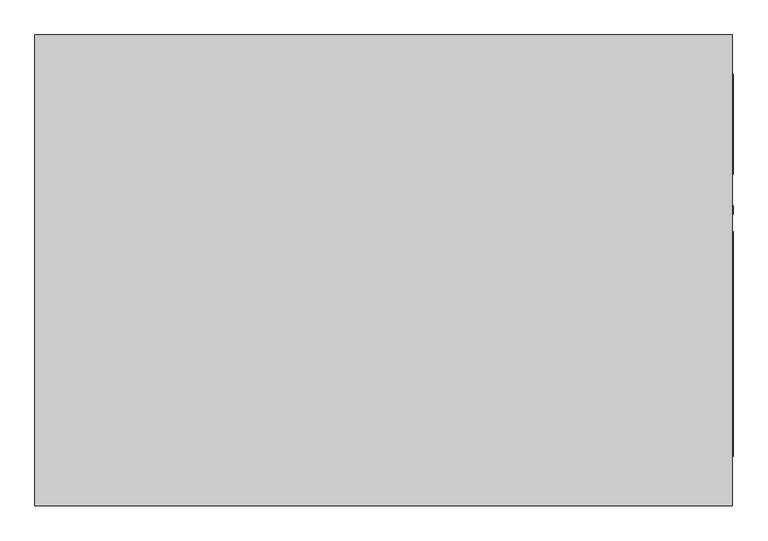
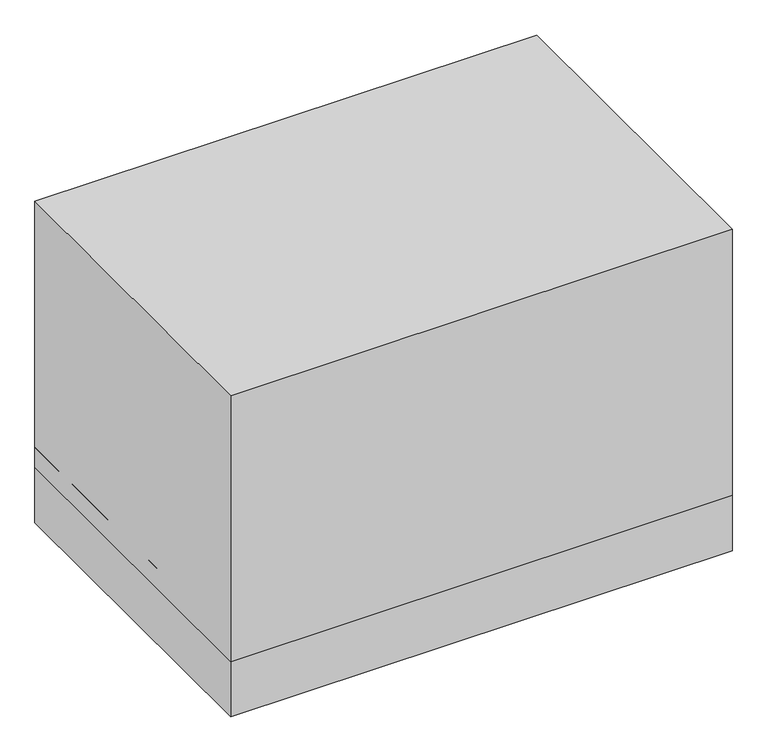
"""IFC4 building model written with IfcOpenShell, lengths in millimetres: proxy geometry, Carrier_48TC_Standard_Efficiency_Gas_Heat_Electric_Cooling_Packaged_Rooftop_Unit_3_to_15_nominal_tons : 12.5 ton 48TC**14."""

import ifcopenshell
import ifcopenshell.guid

model = None  # the IFC model being written
_history = None  # IfcOwnerHistory: only IFC2X3 demands one
_inside = {}  # id of a spatial element -> (the spatial element, [elements in it])
_under = {}  # id of a project, library or spatial element -> (it, [spatial elements below it])
_declared = {}  # id of a project -> (the project, [libraries it declares])
_typed = {}  # id of a type object -> (the type object, [elements of that type])
_made_of = {}  # id of a material, layer set ... -> (it, [elements and type objects made of it])


def new_model(schema):
    """Start an empty IFC model of exactly this schema.

    Asked for "IFC4X3", IfcOpenShell would pick the latest addendum, in which some entities
    have other attributes; the version numbers below select the first issue.
    IFC2X3 requires an IfcOwnerHistory on every rooted entity: one is made here for all.
    """
    global model, _history
    if schema == "IFC4X3":
        model = ifcopenshell.file(schema_version=(4, 3, 0, 0))
    else:
        model = ifcopenshell.file(schema=schema)
    _inside.clear()
    _under.clear()
    _declared.clear()
    _typed.clear()
    _made_of.clear()
    _history = None
    if model.schema == "IFC2X3":
        org = make("IfcOrganization", Name="unknown")
        user = make(
            "IfcPersonAndOrganization",
            ThePerson=make("IfcPerson", FamilyName="unknown"),
            TheOrganization=org,
        )
        app = make(
            "IfcApplication",
            ApplicationDeveloper=org,
            Version="unknown",
            ApplicationFullName="unknown",
            ApplicationIdentifier="unknown",
        )
        _history = make(
            "IfcOwnerHistory",
            OwningUser=user,
            OwningApplication=app,
            ChangeAction="ADDED",
            CreationDate=0,
        )
    return model


def make(cls, **values):
    """One entity of the class cls with the attributes given. An attribute that is None is left unset."""
    return model.create_entity(
        cls, **{name: value for name, value in values.items() if value is not None}
    )


def rooted(cls, **values):
    """An entity with a GlobalId (a new one), such as an element, a storey or a relation."""
    return make(cls, GlobalId=ifcopenshell.guid.new(), OwnerHistory=_history, **values)


def si_unit(unit_type, name, prefix=None):
    """IfcSIUnit, for example si_unit("LENGTHUNIT", "METRE", prefix="MILLI")."""
    return make("IfcSIUnit", UnitType=unit_type, Prefix=prefix, Name=name)


def assignment(units):
    """IfcUnitAssignment: the units of a project."""
    return None if units is None else make("IfcUnitAssignment", Units=units)


def point(xyz):
    """IfcCartesianPoint."""
    return None if xyz is None else make("IfcCartesianPoint", Coordinates=xyz)


def direction(xyz):
    """IfcDirection."""
    return None if xyz is None else make("IfcDirection", DirectionRatios=xyz)


def frame(location, z_axis=None, x_axis=None):
    """IfcAxis2Placement3D, a coordinate frame: its origin and axes. An axis left out is left unset."""
    return make(
        "IfcAxis2Placement3D",
        Location=point(location),
        Axis=direction(z_axis),
        RefDirection=direction(x_axis),
    )


def frame_2d(location, x_axis=None):
    """IfcAxis2Placement2D, a coordinate frame in the plane: its origin and x axis."""
    return make(
        "IfcAxis2Placement2D", Location=point(location), RefDirection=direction(x_axis)
    )


def origin():
    """The frame at (0, 0, 0) with its axes left unset."""
    return frame((0.0, 0.0, 0.0))


def origin_with_axes():
    """The frame at (0, 0, 0) with the z axis (0, 0, 1) and the x axis (1, 0, 0) written out."""
    return frame((0.0, 0.0, 0.0), z_axis=(0.0, 0.0, 1.0), x_axis=(1.0, 0.0, 0.0))


def place(relative_to, where):
    """IfcLocalPlacement: puts the frame where relative to a parent placement (None: the world)."""
    return make(
        "IfcLocalPlacement", PlacementRelTo=relative_to, RelativePlacement=where
    )


def context(
    kind, dimensions, precision=None, world=None, true_north=None, identifier=None
):
    """IfcGeometricRepresentationContext, for example the 3D "Model" context."""
    return make(
        "IfcGeometricRepresentationContext",
        ContextIdentifier=identifier,
        ContextType=kind,
        CoordinateSpaceDimension=dimensions,
        Precision=precision,
        WorldCoordinateSystem=world,
        TrueNorth=true_north,
    )


def project(units=None, contexts=None):
    """IfcProject with its units and contexts."""
    return rooted(
        "IfcProject",
        Name="project",
        RepresentationContexts=contexts,
        UnitsInContext=assignment(units),
    )


def spatial(cls, under=None, at=None, **own):
    """A site, building, storey or space (cls), placed at a placement, below another one or the project."""
    s = rooted(cls, ObjectPlacement=at, **own)
    if under is not None:
        _under.setdefault(under.id(), (under, []))[1].append(s)
    return s


def polyline(points):
    """IfcPolyline through the points."""
    return make("IfcPolyline", Points=[point(p) for p in points])


def circle_curve(where, radius):
    """IfcCircle in the frame where."""
    return make("IfcCircle", Position=where, Radius=radius)


def trimmed(basis, trim1, trim2, sense, master):
    """IfcTrimmedCurve: the piece of a basis curve between two trims."""
    return make(
        "IfcTrimmedCurve",
        BasisCurve=basis,
        Trim1=trim1,
        Trim2=trim2,
        SenseAgreement=sense,
        MasterRepresentation=master,
    )


def segment(curve, same_sense, transition):
    """IfcCompositeCurveSegment."""
    return make(
        "IfcCompositeCurveSegment",
        Transition=transition,
        SameSense=same_sense,
        ParentCurve=curve,
    )


def composite_curve(segments, self_intersect=None):
    """IfcCompositeCurve: segments joined end to end."""
    return make("IfcCompositeCurve", Segments=segments, SelfIntersect=self_intersect)


def outline(outer, holes=None, kind="AREA"):
    """IfcArbitraryClosedProfileDef: a profile drawn as a closed curve; with holes, ...WithVoids."""
    if holes is None:
        return make("IfcArbitraryClosedProfileDef", ProfileType=kind, OuterCurve=outer)
    return make(
        "IfcArbitraryProfileDefWithVoids",
        ProfileType=kind,
        OuterCurve=outer,
        InnerCurves=holes,
    )


def extrude(swept, where, along, depth):
    """IfcExtrudedAreaSolid: the profile swept, set in the frame where, extruded along a direction by depth."""
    return make(
        "IfcExtrudedAreaSolid",
        SweptArea=swept,
        Position=where,
        ExtrudedDirection=direction(along),
        Depth=depth,
    )


def shape(context_of_items, identifier, shape_type, items):
    """IfcShapeRepresentation: the items that make up one representation, for example the "Body"."""
    return make(
        "IfcShapeRepresentation",
        ContextOfItems=context_of_items,
        RepresentationIdentifier=identifier,
        RepresentationType=shape_type,
        Items=items,
    )


def source(mapping_origin, context_of_items, identifier, shape_type, items):
    """IfcRepresentationMap: a shape defined once, which mapped items show again and again."""
    return make(
        "IfcRepresentationMap",
        MappingOrigin=mapping_origin,
        MappedRepresentation=shape(context_of_items, identifier, shape_type, items),
    )


def transform(
    local_origin,
    x_axis=None,
    y_axis=None,
    z_axis=None,
    scale=None,
    scale2=None,
    scale3=None,
    uniform=True,
):
    """IfcCartesianTransformationOperator3D, or its non-uniform kind. x_axis, y_axis, z_axis: its Axis1, 2, 3."""
    if uniform:
        return make(
            "IfcCartesianTransformationOperator3D",
            Axis1=direction(x_axis),
            Axis2=direction(y_axis),
            LocalOrigin=point(local_origin),
            Scale=scale,
            Axis3=direction(z_axis),
        )
    return make(
        "IfcCartesianTransformationOperator3DnonUniform",
        Axis1=direction(x_axis),
        Axis2=direction(y_axis),
        LocalOrigin=point(local_origin),
        Scale=scale,
        Axis3=direction(z_axis),
        Scale2=scale2,
        Scale3=scale3,
    )


def mapped(mapping_source, mapping_target):
    """IfcMappedItem: shows the shape of a source again, moved by a transform."""
    return make(
        "IfcMappedItem", MappingSource=mapping_source, MappingTarget=mapping_target
    )


def made_of(thing, what):
    """Note that an element or type object is made of a material, layer set ...; save() writes the relation."""
    if what is not None:
        _made_of.setdefault(what.id(), (what, []))[1].append(thing)
    return thing


def element(
    cls,
    number,
    at=None,
    inside=None,
    cuts=None,
    type_object=None,
    material=None,
    context=None,
    identifier="Body",
    shape_type=None,
    held_by="IfcProductDefinitionShape",
    body=None,
    shapes=None,
    **own,
):
    """One element of the class cls, such as IfcWall. Its Tag is "e" and its number.

    at: its placement. inside: the storey or other place that contains it. cuts: it is an
    opening in that element (IfcRelVoidsElement). A single representation is given by context,
    identifier, shape_type and body (its items); several are given by shapes. held_by: the class
    of the entity that holds the representations. save() writes the other relations.
    """
    e = rooted(cls, Tag="e%d" % number, ObjectPlacement=at, **own)
    if body is not None:
        shapes = [shape(context, identifier, shape_type, body)]
    if shapes is not None:
        e.Representation = make(held_by, Representations=shapes)
    if inside is not None:
        _inside.setdefault(inside.id(), (inside, []))[1].append(e)
    if cuts is not None:
        rooted(
            "IfcRelVoidsElement", RelatingBuildingElement=cuts, RelatedOpeningElement=e
        )
    if type_object is not None:
        _typed.setdefault(type_object.id(), (type_object, []))[1].append(e)
    return made_of(e, material)


def aggregate(whole, parts):
    """IfcRelAggregates: a whole, such as a stair, and the parts it consists of."""
    return rooted("IfcRelAggregates", RelatingObject=whole, RelatedObjects=parts)


def save(model, path):
    """Write the relations noted so far, then the file.

    IfcRelAggregates (storeys below a building ...), IfcRelContainedInSpatialStructure (elements
    in a storey), IfcRelDefinesByType, IfcRelAssociatesMaterial and IfcRelDeclares: one each for
    every whole, place, type object, material and project.
    """
    for whole, parts in _under.values():
        aggregate(whole, parts)
    for where, things in _inside.values():
        rooted(
            "IfcRelContainedInSpatialStructure",
            RelatedElements=things,
            RelatingStructure=where,
        )
    for kind, things in _typed.values():
        rooted("IfcRelDefinesByType", RelatedObjects=things, RelatingType=kind)
    for what, things in _made_of.values():
        rooted("IfcRelAssociatesMaterial", RelatedObjects=things, RelatingMaterial=what)
    for by, libraries in _declared.values():
        rooted("IfcRelDeclares", RelatingContext=by, RelatedDefinitions=libraries)
    model.write(path)


def plane_surface(at):
    """IfcPlane: the flat surface through the origin of the frame at, square to its z axis."""
    return make("IfcPlane", Position=at)


def revolved_surface(curve, axis_point, axis_direction):
    """IfcSurfaceOfRevolution: the curve turned about the line through axis_point along axis_direction."""
    return make(
        "IfcSurfaceOfRevolution",
        SweptCurve=make("IfcArbitraryOpenProfileDef", ProfileType="CURVE", Curve=curve),
        AxisPosition=make("IfcAxis1Placement", Location=point(axis_point), Axis=direction(axis_direction)),
    )


def advanced_brep(points, edges, surfaces, faces):
    """IfcAdvancedBrep: a solid bounded by faces that lie on surfaces and meet in shared edges.

    An edge is (start, end): straight between two places in points (the first is 0);
    or (start, end, curve); or (start, end, curve, False) where it runs against its curve.
    A face is (place in surfaces, loops), or (place, loops, False) where it looks against
    its surface's normal. A loop lists edges by number (the first is 1), with a minus sign
    where the edge is run from its end to its start. The first loop is the outer one.
    """
    corners = [point(p) for p in points]
    vertices = [make("IfcVertexPoint", VertexGeometry=c) for c in corners]
    made = []
    for start, end, *more in edges:
        made.append(
            make(
                "IfcEdgeCurve",
                EdgeStart=vertices[start],
                EdgeEnd=vertices[end],
                EdgeGeometry=more[0] if more else make("IfcPolyline", Points=[corners[start], corners[end]]),
                SameSense=more[1] if len(more) > 1 else True,
            )
        )
    hull = []
    for where, loops, *sense in faces:
        bounds = []
        for j, loop in enumerate(loops):
            ring = [make("IfcOrientedEdge", EdgeElement=made[abs(k) - 1], Orientation=k > 0) for k in loop]
            bounds.append(
                make(
                    "IfcFaceOuterBound" if j == 0 else "IfcFaceBound",
                    Bound=make("IfcEdgeLoop", EdgeList=ring),
                    Orientation=True,
                )
            )
        hull.append(make("IfcAdvancedFace", Bounds=bounds, FaceSurface=surfaces[where], SameSense=sense[0] if sense else True))
    return make("IfcAdvancedBrep", Outer=make("IfcClosedShell", CfsFaces=hull))


def mechanical_equipment_3d4f0b1e(model_context):
    return source(origin(), model_context, "Body", "SolidModel", [
        extrude(outline(composite_curve([segment(trimmed(circle_curve(frame_2d((193.675, 438.15)), 13.2953125), [point((180.3796875, 438.15))], [point((206.9703125, 438.15))], False, "CARTESIAN"), True, "CONTINUOUS"), segment(trimmed(circle_curve(frame_2d((193.675, 438.15)), 13.2953125), [point((206.9703125, 438.15))], [point((180.3796875, 438.15))], False, "CARTESIAN"), True, "CONTINUOUS")], self_intersect=False)), frame((1119.1875, 0.0, 0.0), z_axis=(1.0, 0.0, 0.0), x_axis=(0.0, 1.0, 0.0)), (0.0, 0.0, 1.0), 3.175),
        advanced_brep(
        [(1119.1875, 755.65, 1514.475), (-1119.1875, 755.65, 1514.475), (-1119.1875, -755.65, 1514.475), (1119.1875, -755.65, 1514.475), (1119.1875, 755.65, 260.35), (1119.1875, -755.65, 260.35), (-1119.1875, -755.65, 260.35), (-1119.1875, 755.65, 260.35), (1036.6375, -596.9, 260.35), (1036.6375, 0.0, 260.35), (681.0375, 0.0, 260.35), (681.0375, -596.9, 260.35), (1036.6375, 590.55, 260.35), (112.7125, 590.55, 260.35), (112.7125, 269.875, 260.35), (1036.6375, 269.875, 260.35), (176.8078125, -107.95, 260.35), (150.2171875, -107.95, 260.35), (-355.6, -476.25, 260.35), (-377.825, -476.25, 260.35), (-344.4875, -349.25, 260.35), (-388.9375, -349.25, 260.35), (-344.4875, -298.45, 260.35), (-388.9375, -298.45, 260.35), (1036.6375, -596.9, 381.0), (681.0375, -596.9, 381.0), (681.0375, 0.0, 381.0), (1036.6375, 0.0, 381.0), (1036.6375, 590.55, 381.0), (1036.6375, 269.875, 381.0), (112.7125, 269.875, 381.0), (112.7125, 590.55, 381.0), (176.8078125, -107.95, 406.4), (150.2171875, -107.95, 406.4), (-355.6, -476.25, 406.4), (-377.825, -476.25, 406.4), (-344.4875, -349.25, 406.4), (-388.9375, -349.25, 406.4), (-344.4875, -298.45, 406.4), (-388.9375, -298.45, 406.4)],
        [
            (0, 1),
            (1, 2),
            (2, 3),
            (3, 0),
            (4, 5),
            (5, 6),
            (6, 7),
            (7, 4),
            (8, 9),
            (9, 10),
            (10, 11),
            (11, 8),
            (12, 13),
            (13, 14),
            (14, 15),
            (15, 12),
            (16, 17, circle_curve(frame((163.5125, -107.95, 260.35), z_axis=(0.0, 0.0, 1.0), x_axis=(-1.0, 0.0, 0.0)), 13.2953125)),
            (17, 16, circle_curve(frame((163.5125, -107.95, 260.35), z_axis=(0.0, 0.0, 1.0), x_axis=(-1.0, 0.0, 0.0)), 13.2953125)),
            (18, 19, circle_curve(frame((-366.7125, -476.25, 260.35), z_axis=(0.0, 0.0, 1.0), x_axis=(-1.0, 0.0, 0.0)), 11.1125)),
            (19, 18, circle_curve(frame((-366.7125, -476.25, 260.35), z_axis=(0.0, 0.0, 1.0), x_axis=(-1.0, 0.0, 0.0)), 11.1125)),
            (20, 21, circle_curve(frame((-366.7125, -349.25, 260.35), z_axis=(0.0, 0.0, 1.0), x_axis=(-1.0, 0.0, 0.0)), 22.225)),
            (21, 20, circle_curve(frame((-366.7125, -349.25, 260.35), z_axis=(0.0, 0.0, 1.0), x_axis=(-1.0, 0.0, 0.0)), 22.225)),
            (22, 23, circle_curve(frame((-366.7125, -298.45, 260.35), z_axis=(0.0, 0.0, 1.0), x_axis=(-1.0, 0.0, 0.0)), 22.225)),
            (23, 22, circle_curve(frame((-366.7125, -298.45, 260.35), z_axis=(0.0, 0.0, 1.0), x_axis=(-1.0, 0.0, 0.0)), 22.225)),
            (0, 4),
            (7, 1),
            (6, 2),
            (5, 3),
            (24, 25),
            (25, 26),
            (26, 27),
            (27, 24),
            (27, 9),
            (8, 24),
            (26, 10),
            (25, 11),
            (28, 29),
            (29, 30),
            (30, 31),
            (31, 28),
            (31, 13),
            (12, 28),
            (30, 14),
            (29, 15),
            (32, 33, circle_curve(frame((163.5125, -107.95, 406.4), z_axis=(0.0, 0.0, -1.0), x_axis=(-1.0, 0.0, 0.0)), 13.2953125)),
            (33, 32, circle_curve(frame((163.5125, -107.95, 406.4), z_axis=(0.0, 0.0, -1.0), x_axis=(-1.0, 0.0, 0.0)), 13.2953125)),
            (33, 17),
            (16, 32),
            (34, 35, circle_curve(frame((-366.7125, -476.25, 406.4), z_axis=(0.0, 0.0, -1.0), x_axis=(-1.0, 0.0, 0.0)), 11.1125)),
            (35, 34, circle_curve(frame((-366.7125, -476.25, 406.4), z_axis=(0.0, 0.0, -1.0), x_axis=(-1.0, 0.0, 0.0)), 11.1125)),
            (35, 19),
            (18, 34),
            (36, 37, circle_curve(frame((-366.7125, -349.25, 406.4), z_axis=(0.0, 0.0, -1.0), x_axis=(-1.0, 0.0, 0.0)), 22.225)),
            (37, 36, circle_curve(frame((-366.7125, -349.25, 406.4), z_axis=(0.0, 0.0, -1.0), x_axis=(-1.0, 0.0, 0.0)), 22.225)),
            (37, 21),
            (20, 36),
            (38, 39, circle_curve(frame((-366.7125, -298.45, 406.4), z_axis=(0.0, 0.0, -1.0), x_axis=(-1.0, 0.0, 0.0)), 22.225)),
            (39, 38, circle_curve(frame((-366.7125, -298.45, 406.4), z_axis=(0.0, 0.0, -1.0), x_axis=(-1.0, 0.0, 0.0)), 22.225)),
            (39, 23),
            (22, 38),
        ],
        [
            plane_surface(frame((-1119.1875, 755.65, 1514.475), z_axis=(0.0, 0.0, 1.0), x_axis=(-1.0, 0.0, 0.0))),
            plane_surface(frame((-1119.1875, 755.65, 260.35), z_axis=(0.0, 0.0, -1.0), x_axis=(1.0, 0.0, 0.0))),
            plane_surface(frame((1119.1875, 755.65, 1514.475), z_axis=(0.0, 1.0, 0.0), x_axis=(0.0, 0.0, -1.0))),
            plane_surface(frame((-1119.1875, 755.65, 1514.475), z_axis=(-1.0, 0.0, 0.0), x_axis=(0.0, 0.0, -1.0))),
            plane_surface(frame((-1119.1875, -755.65, 1514.475), z_axis=(0.0, -1.0, 0.0), x_axis=(0.0, 0.0, -1.0))),
            plane_surface(frame((1119.1875, -755.65, 1514.475), z_axis=(1.0, 0.0, 0.0), x_axis=(0.0, 0.0, -1.0))),
            plane_surface(frame((1036.6375, -596.9, 381.0), z_axis=(0.0, 0.0, -1.0), x_axis=(0.0, 1.0, 0.0))),
            plane_surface(frame((1036.6375, -596.9, 381.0), z_axis=(-1.0, 0.0, 0.0), x_axis=(0.0, 0.0, -1.0))),
            plane_surface(frame((1036.6375, 0.0, 381.0), z_axis=(0.0, -1.0, 0.0), x_axis=(0.0, 0.0, -1.0))),
            plane_surface(frame((681.0375, 0.0, 381.0), z_axis=(1.0, 0.0, 0.0), x_axis=(0.0, 0.0, -1.0))),
            plane_surface(frame((681.0375, -596.9, 381.0), z_axis=(0.0, 1.0, 0.0), x_axis=(0.0, 0.0, -1.0))),
            plane_surface(frame((112.7125, 590.55, 381.0), z_axis=(0.0, 0.0, -1.0), x_axis=(-1.0, 0.0, 0.0))),
            plane_surface(frame((1036.6375, 590.55, 381.0), z_axis=(0.0, -1.0, 0.0), x_axis=(0.0, 0.0, -1.0))),
            plane_surface(frame((112.7125, 590.55, 381.0), z_axis=(1.0, 0.0, 0.0), x_axis=(0.0, 0.0, -1.0))),
            plane_surface(frame((112.7125, 269.875, 381.0), z_axis=(0.0, 1.0, 0.0), x_axis=(0.0, 0.0, -1.0))),
            plane_surface(frame((1036.6375, 269.875, 381.0), z_axis=(-1.0, 0.0, 0.0), x_axis=(0.0, 0.0, -1.0))),
            plane_surface(frame((150.2171875, -107.95, 406.4), z_axis=(0.0, 0.0, -1.0), x_axis=(0.0, -1.0, 0.0))),
            revolved_surface(polyline([(150.2171875, -107.95, 406.4), (150.2171875, -107.95, 260.35)]), (163.5125, -107.95, 0.0), (0.0, 0.0, 1.0)),
            plane_surface(frame((-377.825, -476.25, 406.4), z_axis=(0.0, 0.0, -1.0), x_axis=(0.0, -1.0, 0.0))),
            revolved_surface(polyline([(-377.825, -476.25, 406.4), (-377.825, -476.25, 260.35)]), (-366.7125, -476.25, 0.0), (0.0, 0.0, 1.0)),
            plane_surface(frame((-388.9375, -349.25, 406.4), z_axis=(0.0, 0.0, -1.0), x_axis=(0.0, -1.0, 0.0))),
            revolved_surface(polyline([(-388.9375, -349.25, 406.4), (-388.9375, -349.25, 260.35)]), (-366.7125, -349.25, 0.0), (0.0, 0.0, 1.0)),
            plane_surface(frame((-388.9375, -298.45, 406.4), z_axis=(0.0, 0.0, -1.0), x_axis=(0.0, -1.0, 0.0))),
            revolved_surface(polyline([(-388.9375, -298.45, 406.4), (-388.9375, -298.45, 260.35)]), (-366.7125, -298.45, 0.0), (0.0, 0.0, 1.0)),
        ],
        [
            (0, [[1, 2, 3, 4]]),
            (1, [[5, 6, 7, 8], [9, 10, 11, 12], [13, 14, 15, 16], [17, 18], [19, 20], [21, 22], [23, 24]]),
            (2, [[-1, 25, -8, 26]]),
            (3, [[-2, -26, -7, 27]]),
            (4, [[-3, -27, -6, 28]]),
            (5, [[-4, -28, -5, -25]]),
            (6, [[29, 30, 31, 32]]),
            (7, [[-32, 33, -9, 34]]),
            (8, [[-31, 35, -10, -33]]),
            (9, [[-30, 36, -11, -35]]),
            (10, [[-29, -34, -12, -36]]),
            (11, [[37, 38, 39, 40]]),
            (12, [[-40, 41, -13, 42]]),
            (13, [[-39, 43, -14, -41]]),
            (14, [[-38, 44, -15, -43]]),
            (15, [[-37, -42, -16, -44]]),
            (16, [[45, 46]]),
            (17, [[-46, 47, -17, 48]]),
            (17, [[-45, -48, -18, -47]]),
            (18, [[49, 50]]),
            (19, [[-50, 51, -19, 52]]),
            (19, [[-49, -52, -20, -51]]),
            (20, [[53, 54]]),
            (21, [[-54, 55, -21, 56]]),
            (21, [[-53, -56, -22, -55]]),
            (22, [[57, 58]]),
            (23, [[-58, 59, -23, 60]]),
            (23, [[-57, -60, -24, -59]]),
        ],
    ),
        extrude(outline(polyline([(1119.1875, 755.65), (1119.1875, -755.65), (-1119.1875, -755.65), (-1119.1875, 755.65), (1119.1875, 755.65)]), holes=[polyline([(1036.6375, 590.55), (112.7125, 590.55), (112.7125, 269.875), (1036.6375, 269.875), (1036.6375, 590.55)]), polyline([(1036.6375, -596.9), (1036.6375, 0.0), (681.0375, 0.0), (681.0375, -596.9), (1036.6375, -596.9)]), composite_curve([segment(trimmed(circle_curve(frame_2d((163.5125, -107.95)), 13.2953125), [point((176.8078125, -107.95))], [point((150.2171875, -107.95))], True, "CARTESIAN"), True, "CONTINUOUS"), segment(trimmed(circle_curve(frame_2d((163.5125, -107.95)), 13.2953125), [point((150.2171875, -107.95))], [point((176.8078125, -107.95))], True, "CARTESIAN"), True, "CONTINUOUS")], self_intersect=False), composite_curve([segment(trimmed(circle_curve(frame_2d((-366.7125, -476.25)), 11.1125), [point((-355.6, -476.25))], [point((-377.825, -476.25))], True, "CARTESIAN"), True, "CONTINUOUS"), segment(trimmed(circle_curve(frame_2d((-366.7125, -476.25)), 11.1125), [point((-377.825, -476.25))], [point((-355.6, -476.25))], True, "CARTESIAN"), True, "CONTINUOUS")], self_intersect=False), composite_curve([segment(trimmed(circle_curve(frame_2d((-366.7125, -349.25)), 22.225), [point((-344.4875, -349.25))], [point((-388.9375, -349.25))], True, "CARTESIAN"), True, "CONTINUOUS"), segment(trimmed(circle_curve(frame_2d((-366.7125, -349.25)), 22.225), [point((-388.9375, -349.25))], [point((-344.4875, -349.25))], True, "CARTESIAN"), True, "CONTINUOUS")], self_intersect=False), composite_curve([segment(trimmed(circle_curve(frame_2d((-366.7125, -298.45)), 22.225), [point((-344.4875, -298.45))], [point((-388.9375, -298.45))], True, "CARTESIAN"), True, "CONTINUOUS"), segment(trimmed(circle_curve(frame_2d((-366.7125, -298.45)), 22.225), [point((-388.9375, -298.45))], [point((-344.4875, -298.45))], True, "CARTESIAN"), True, "CONTINUOUS")], self_intersect=False)]), origin_with_axes(), (0.0, 0.0, 1.0), 355.6),
        extrude(outline(polyline([(1122.3625, 628.65), (1122.3625, 307.975), (1119.1875, 307.975), (1119.1875, 628.65), (1122.3625, 628.65)])), frame((0.0, 0.0, 406.4), z_axis=(0.0, 0.0, 1.0), x_axis=(1.0, 0.0, 0.0)), (0.0, 0.0, 1.0), 923.925),
        extrude(outline(polyline([(1122.3625, 123.825), (1122.3625, -596.9), (1119.1875, -596.9), (1119.1875, 123.825), (1122.3625, 123.825)])), frame((0.0, 0.0, 406.4), z_axis=(0.0, 0.0, 1.0), x_axis=(1.0, 0.0, 0.0)), (0.0, 0.0, 1.0), 352.425),
    ])


if __name__ == "__main__":
    model = new_model("IFC4")
    model_context = context("Model", 3, world=origin())
    ifc_project = project(units=[si_unit("LENGTHUNIT", "METRE", prefix="MILLI")], contexts=[model_context])
    site = spatial("IfcSite", under=ifc_project)
    building = spatial("IfcBuilding", under=site)
    placement = place(None, origin())
    mechanical_equipment_shape = mechanical_equipment_3d4f0b1e(model_context)
    element("IfcBuildingElementProxy", 1, Name="Carrier_48TC_Standard_Efficiency_Gas_Heat_Electric_Cooling_Packaged_Rooftop_Unit_3_to_15_nominal_tons : 12.5 ton 48TC**14", ObjectType="Carrier_48TC_Standard_Efficiency_Gas_Heat_Electric_Cooling_Packaged_Rooftop_Unit_3_to_15_nominal_tons : 12.5 ton 48TC**14", at=placement, inside=building, context=model_context, shape_type="MappedRepresentation", body=[
        mapped(mechanical_equipment_shape, transform((0.0, 0.0, 0.0), x_axis=(1.0, 0.0, 0.0), y_axis=(0.0, 1.0, 0.0), z_axis=(0.0, 0.0, 1.0))),
    ])
    save(model, "model.ifc")

# Revit data of these elements
# Type "Carrier_48TC_Standard_Efficiency_Gas_Heat_Electric_Cooling_Packaged_Rooftop_Unit_3_to_15_nominal_tons : 12.5 ton 48TC**14"
#   URL = "www.Carrier.com"
#   Model = "48TC"
#   Manufacturer = "Carrier"
#   Disclaimer = "Manufacturer reserves the right to change, at any time, specifications and designs without notice and without obligation.  Please verify critical parameters with local Carrier commercial sales office."
#   knockout thickness = 0' - 0 1/16"
#   Voltage = 0 V
#   Version = 1
#   TTBY3 = 0' - 11"
#   TTBY2 = 1' - 4"
#   TTBY1 = 1' - 6"
#   TTBX = 2' - 5 5/8"
#   TTBPowerR = 0' - 0 7/8"
#   TTBGasR = 0' - 0 7/8"
#   SSSZ = 0' - 5 3/4"
#   SSSY = 0' - 6 1/4"
#   SSSW = 2' - 4 3/8"
#   SSSH = 1' - 1 7/8"
#   SSRZ = 0' - 5 3/4"
#   SSRY = 0' - 5"
#   SSRW = 1' - 0 5/8"
#   SSRH = 3' - 0 3/8"
#   SEER = 0
#   Right clearance = 3' - 0"
#   PWRZ = 3' - 0"
#   PWRY = 0' - 4 5/8"
#   PWRR = 0' - 1 1/4"
#   ODF2X = 1' - 0"
#   ODF1Y = 1' - 7"
#   ODF1X = 1' - 7"
#   ODF1R = 1' - 6"
#   MOCP = 0 A
#   MCA = 0 A
#   Left clearance = 4' - 0"
#   IEER = 11
#   Front clearance = 4' - 0"
#   Fan Z = 4' - 11 5/8"
#   Width = 4' - 11 1/2"
#   Length = 7' - 4 1/8"
#   Height = 4' - 1 3/8"
#   EER = 10.8
#   DSSY = 0' - 6 1/4"
#   DSSX = 0' - 3 1/4"
#   DSSW = 1' - 2"
#   DSSH = 2' - 4 3/4"
#   DSRY = 0' - 6 1/2"
#   DSRX = 0' - 3 1/4"
#   DSRW = 3' - 0 3/8"
#   DSRH = 1' - 0 5/8"
#   DRNZ = 0' - 7"
#   DRNY = 3' - 1 3/8"
#   DRNR = 0' - 0 67/128"
#   Curb Z = 1' - 2"
#   CFM (nominal) = 0 CFM
#   Back clearance = 3' - 0"
#   Alt Condensate Drain = 0' - 0 67/128"
#   AccypwrR = 0' - 0 7/16"
#   ACY = 2' - 1 1/2"
#   ACX = 3' - 1 5/8"
#   Gas [instance default] = yes
#   Fan 2 on = no
#   Curb_1SLAB_2ROOFCURB_3SNOWCURB = 2
#   Fan 3 on = no
#   Unit material = SINGLE-PACKAGED ROOFTOP UNITS
#   Curb material = Curb paint
# Element 1 (IfcBuildingElementProxy, "Carrier_48TC_Standard_Efficiency_Gas_Heat_Electric_Cooling_Packaged_Rooftop_Unit_3_to_15_nominal_tons : 12.5 ton 48TC**14")
#   Materials on its faces: "SINGLE-PACKAGED ROOFTOP UNITS", "Curb paint", "Mech"
# Materials
#   "SINGLE-PACKAGED ROOFTOP UNITS": class "Miscellaneous", colour RGB 201 201 201, transparency 0, Cost = 0
#   "Curb paint": class "Miscellaneous", colour RGB 189 187 185, transparency 0
#   "Mech": class "Miscellaneous", colour RGB 235 237 235, transparency 0, Cost = 0
